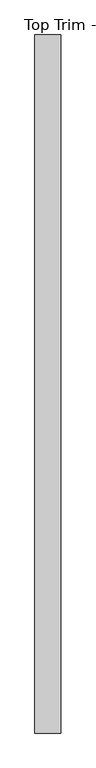
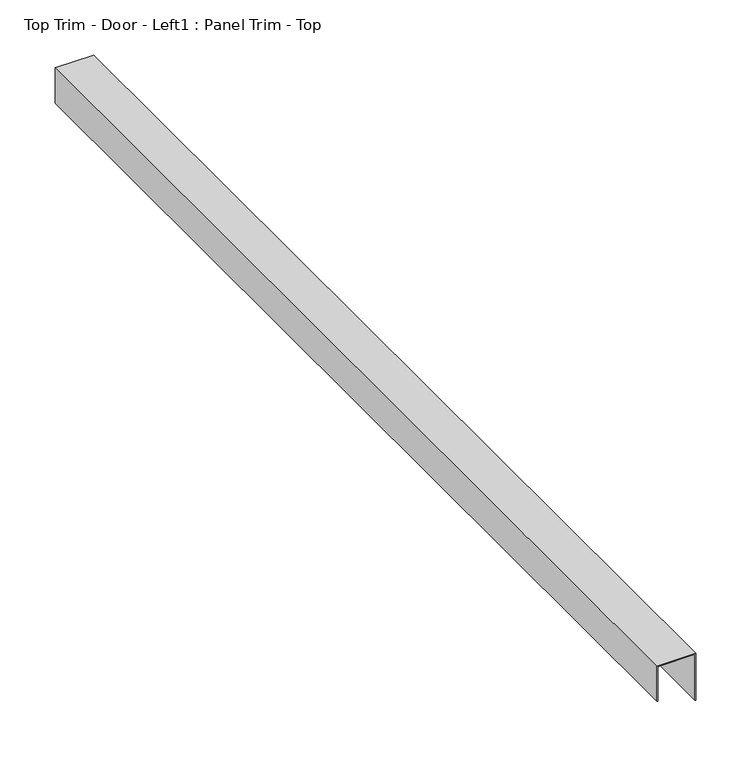
"""IFC4 building model written with IfcOpenShell, lengths in millimetres: proxy geometry, Top Trim - Door - Left1 : Panel Trim - Top."""

import ifcopenshell
import ifcopenshell.guid

model = None  # the IFC model being written
_history = None  # IfcOwnerHistory: only IFC2X3 demands one
_inside = {}  # id of a spatial element -> (the spatial element, [elements in it])
_under = {}  # id of a project, library or spatial element -> (it, [spatial elements below it])
_declared = {}  # id of a project -> (the project, [libraries it declares])
_typed = {}  # id of a type object -> (the type object, [elements of that type])
_made_of = {}  # id of a material, layer set ... -> (it, [elements and type objects made of it])


def new_model(schema):
    """Start an empty IFC model of exactly this schema.

    Asked for "IFC4X3", IfcOpenShell would pick the latest addendum, in which some entities
    have other attributes; the version numbers below select the first issue.
    IFC2X3 requires an IfcOwnerHistory on every rooted entity: one is made here for all.
    """
    global model, _history
    if schema == "IFC4X3":
        model = ifcopenshell.file(schema_version=(4, 3, 0, 0))
    else:
        model = ifcopenshell.file(schema=schema)
    _inside.clear()
    _under.clear()
    _declared.clear()
    _typed.clear()
    _made_of.clear()
    _history = None
    if model.schema == "IFC2X3":
        org = make("IfcOrganization", Name="unknown")
        user = make(
            "IfcPersonAndOrganization",
            ThePerson=make("IfcPerson", FamilyName="unknown"),
            TheOrganization=org,
        )
        app = make(
            "IfcApplication",
            ApplicationDeveloper=org,
            Version="unknown",
            ApplicationFullName="unknown",
            ApplicationIdentifier="unknown",
        )
        _history = make(
            "IfcOwnerHistory",
            OwningUser=user,
            OwningApplication=app,
            ChangeAction="ADDED",
            CreationDate=0,
        )
    return model


def make(cls, **values):
    """One entity of the class cls with the attributes given. An attribute that is None is left unset."""
    return model.create_entity(
        cls, **{name: value for name, value in values.items() if value is not None}
    )


def rooted(cls, **values):
    """An entity with a GlobalId (a new one), such as an element, a storey or a relation."""
    return make(cls, GlobalId=ifcopenshell.guid.new(), OwnerHistory=_history, **values)


def si_unit(unit_type, name, prefix=None):
    """IfcSIUnit, for example si_unit("LENGTHUNIT", "METRE", prefix="MILLI")."""
    return make("IfcSIUnit", UnitType=unit_type, Prefix=prefix, Name=name)


def assignment(units):
    """IfcUnitAssignment: the units of a project."""
    return None if units is None else make("IfcUnitAssignment", Units=units)


def point(xyz):
    """IfcCartesianPoint."""
    return None if xyz is None else make("IfcCartesianPoint", Coordinates=xyz)


def direction(xyz):
    """IfcDirection."""
    return None if xyz is None else make("IfcDirection", DirectionRatios=xyz)


def frame(location, z_axis=None, x_axis=None):
    """IfcAxis2Placement3D, a coordinate frame: its origin and axes. An axis left out is left unset."""
    return make(
        "IfcAxis2Placement3D",
        Location=point(location),
        Axis=direction(z_axis),
        RefDirection=direction(x_axis),
    )


def origin():
    """The frame at (0, 0, 0) with its axes left unset."""
    return frame((0.0, 0.0, 0.0))


def place(relative_to, where):
    """IfcLocalPlacement: puts the frame where relative to a parent placement (None: the world)."""
    return make(
        "IfcLocalPlacement", PlacementRelTo=relative_to, RelativePlacement=where
    )


def context(
    kind, dimensions, precision=None, world=None, true_north=None, identifier=None
):
    """IfcGeometricRepresentationContext, for example the 3D "Model" context."""
    return make(
        "IfcGeometricRepresentationContext",
        ContextIdentifier=identifier,
        ContextType=kind,
        CoordinateSpaceDimension=dimensions,
        Precision=precision,
        WorldCoordinateSystem=world,
        TrueNorth=true_north,
    )


def project(units=None, contexts=None):
    """IfcProject with its units and contexts."""
    return rooted(
        "IfcProject",
        Name="project",
        RepresentationContexts=contexts,
        UnitsInContext=assignment(units),
    )


def spatial(cls, under=None, at=None, **own):
    """A site, building, storey or space (cls), placed at a placement, below another one or the project."""
    s = rooted(cls, ObjectPlacement=at, **own)
    if under is not None:
        _under.setdefault(under.id(), (under, []))[1].append(s)
    return s


def polyline(points):
    """IfcPolyline through the points."""
    return make("IfcPolyline", Points=[point(p) for p in points])


def outline(outer, holes=None, kind="AREA"):
    """IfcArbitraryClosedProfileDef: a profile drawn as a closed curve; with holes, ...WithVoids."""
    if holes is None:
        return make("IfcArbitraryClosedProfileDef", ProfileType=kind, OuterCurve=outer)
    return make(
        "IfcArbitraryProfileDefWithVoids",
        ProfileType=kind,
        OuterCurve=outer,
        InnerCurves=holes,
    )


def extrude(swept, where, along, depth):
    """IfcExtrudedAreaSolid: the profile swept, set in the frame where, extruded along a direction by depth."""
    return make(
        "IfcExtrudedAreaSolid",
        SweptArea=swept,
        Position=where,
        ExtrudedDirection=direction(along),
        Depth=depth,
    )


def shape(context_of_items, identifier, shape_type, items):
    """IfcShapeRepresentation: the items that make up one representation, for example the "Body"."""
    return make(
        "IfcShapeRepresentation",
        ContextOfItems=context_of_items,
        RepresentationIdentifier=identifier,
        RepresentationType=shape_type,
        Items=items,
    )


def source(mapping_origin, context_of_items, identifier, shape_type, items):
    """IfcRepresentationMap: a shape defined once, which mapped items show again and again."""
    return make(
        "IfcRepresentationMap",
        MappingOrigin=mapping_origin,
        MappedRepresentation=shape(context_of_items, identifier, shape_type, items),
    )


def transform(
    local_origin,
    x_axis=None,
    y_axis=None,
    z_axis=None,
    scale=None,
    scale2=None,
    scale3=None,
    uniform=True,
):
    """IfcCartesianTransformationOperator3D, or its non-uniform kind. x_axis, y_axis, z_axis: its Axis1, 2, 3."""
    if uniform:
        return make(
            "IfcCartesianTransformationOperator3D",
            Axis1=direction(x_axis),
            Axis2=direction(y_axis),
            LocalOrigin=point(local_origin),
            Scale=scale,
            Axis3=direction(z_axis),
        )
    return make(
        "IfcCartesianTransformationOperator3DnonUniform",
        Axis1=direction(x_axis),
        Axis2=direction(y_axis),
        LocalOrigin=point(local_origin),
        Scale=scale,
        Axis3=direction(z_axis),
        Scale2=scale2,
        Scale3=scale3,
    )


def mapped(mapping_source, mapping_target):
    """IfcMappedItem: shows the shape of a source again, moved by a transform."""
    return make(
        "IfcMappedItem", MappingSource=mapping_source, MappingTarget=mapping_target
    )


def made_of(thing, what):
    """Note that an element or type object is made of a material, layer set ...; save() writes the relation."""
    if what is not None:
        _made_of.setdefault(what.id(), (what, []))[1].append(thing)
    return thing


def element(
    cls,
    number,
    at=None,
    inside=None,
    cuts=None,
    type_object=None,
    material=None,
    context=None,
    identifier="Body",
    shape_type=None,
    held_by="IfcProductDefinitionShape",
    body=None,
    shapes=None,
    **own,
):
    """One element of the class cls, such as IfcWall. Its Tag is "e" and its number.

    at: its placement. inside: the storey or other place that contains it. cuts: it is an
    opening in that element (IfcRelVoidsElement). A single representation is given by context,
    identifier, shape_type and body (its items); several are given by shapes. held_by: the class
    of the entity that holds the representations. save() writes the other relations.
    """
    e = rooted(cls, Tag="e%d" % number, ObjectPlacement=at, **own)
    if body is not None:
        shapes = [shape(context, identifier, shape_type, body)]
    if shapes is not None:
        e.Representation = make(held_by, Representations=shapes)
    if inside is not None:
        _inside.setdefault(inside.id(), (inside, []))[1].append(e)
    if cuts is not None:
        rooted(
            "IfcRelVoidsElement", RelatingBuildingElement=cuts, RelatedOpeningElement=e
        )
    if type_object is not None:
        _typed.setdefault(type_object.id(), (type_object, []))[1].append(e)
    return made_of(e, material)


def aggregate(whole, parts):
    """IfcRelAggregates: a whole, such as a stair, and the parts it consists of."""
    return rooted("IfcRelAggregates", RelatingObject=whole, RelatedObjects=parts)


def save(model, path):
    """Write the relations noted so far, then the file.

    IfcRelAggregates (storeys below a building ...), IfcRelContainedInSpatialStructure (elements
    in a storey), IfcRelDefinesByType, IfcRelAssociatesMaterial and IfcRelDeclares: one each for
    every whole, place, type object, material and project.
    """
    for whole, parts in _under.values():
        aggregate(whole, parts)
    for where, things in _inside.values():
        rooted(
            "IfcRelContainedInSpatialStructure",
            RelatedElements=things,
            RelatingStructure=where,
        )
    for kind, things in _typed.values():
        rooted("IfcRelDefinesByType", RelatedObjects=things, RelatingType=kind)
    for what, things in _made_of.values():
        rooted("IfcRelAssociatesMaterial", RelatedObjects=things, RelatingMaterial=what)
    for by, libraries in _declared.values():
        rooted("IfcRelDeclares", RelatingContext=by, RelatedDefinitions=libraries)
    model.write(path)


def top_trim_door_left1_panel_trim_top_50f9c082(model_context):
    return source(origin(), model_context, "Body", "SweptSolid", [
        extrude(outline(polyline([(2438.4, 587327.0060739), (2438.4, 587365.8934739), (2387.6, 587365.8934739), (2387.6, 587366.6808739), (2439.19375, 587366.6808739), (2439.19375, 587326.2186739), (2400.3, 587326.2186739), (2400.3, 587327.0060739), (2438.4, 587327.0060739)])), frame((0.0, -535201.5663841, 0.0), z_axis=(0.0, 1.0, 0.0), x_axis=(0.0, 0.0, 1.0)), (0.0, 0.0, 1.0), 1092.2),
    ])


if __name__ == "__main__":
    model = new_model("IFC4")
    model_context = context("Model", 3, world=origin())
    ifc_project = project(units=[si_unit("LENGTHUNIT", "METRE", prefix="MILLI")], contexts=[model_context])
    site = spatial("IfcSite", under=ifc_project)
    building = spatial("IfcBuilding", under=site)
    placement = place(None, origin())
    top_trim_door_left1_panel_trim_top_shape = top_trim_door_left1_panel_trim_top_50f9c082(model_context)
    element("IfcBuildingElementProxy", 1, Name="Top Trim - Door - Left1 : Panel Trim - Top", ObjectType="Top Trim - Door - Left1 : Panel Trim - Top", at=placement, inside=building, context=model_context, shape_type="MappedRepresentation", body=[
        mapped(top_trim_door_left1_panel_trim_top_shape, transform((0.0, 0.0, 0.0), x_axis=(1.0, 0.0, 0.0), y_axis=(0.0, 1.0, 0.0), z_axis=(0.0, 0.0, 1.0))),
    ])
    save(model, "model.ifc")

# Revit data of these elements
# Element 1 (IfcBuildingElementProxy, "Top Trim - Door - Left1 : Panel Trim - Top")
#   Materials on its faces: "EDGE TRIM BY MTL PANEL MFR."
# Materials
#   "EDGE TRIM BY MTL PANEL MFR.": class "Generic", colour RGB 239 242 240, transparency 0, Cost = 0
